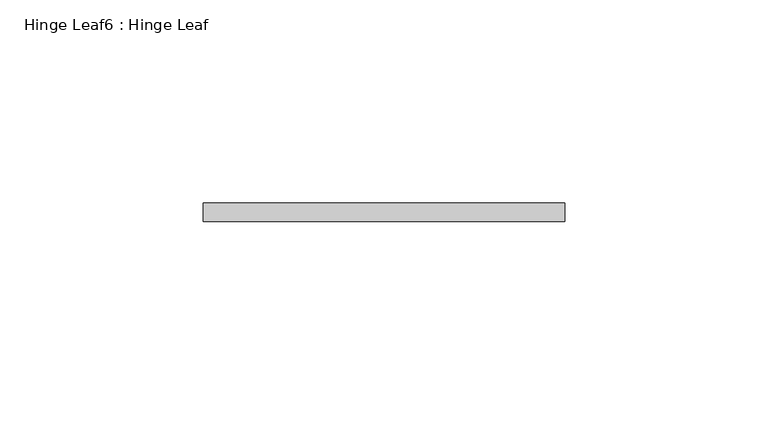
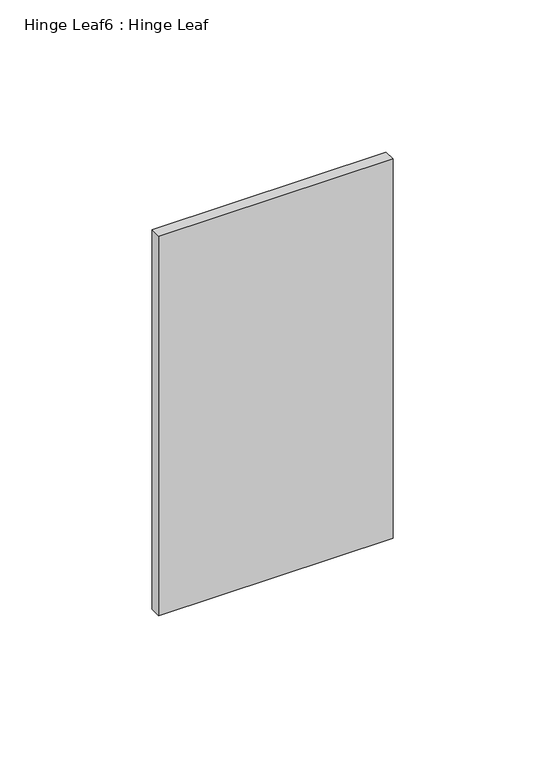
"""IFC4 building model written with IfcOpenShell, lengths in millimetres: proxy geometry, Hinge Leaf6 : Hinge Leaf."""

from ifc_helpers import new_model, si_unit, frame, origin, place, context, project, spatial, polyline, outline, extrude, source, transform, mapped, element, save


def hinge_leaf6_hinge_leaf_bcfbb292(model_context):
    return source(origin(), model_context, "Body", "SweptSolid", [
        extrude(outline(polyline([(587327.7934739, -533980.5883841), (587327.7934739, -533976.0163841), (587416.6934739, -533976.0163841), (587416.6934739, -533980.5883841), (587327.7934739, -533980.5883841)])), frame((0.0, 0.0, 311.15), z_axis=(0.0, 0.0, 1.0), x_axis=(1.0, 0.0, 0.0)), (0.0, 0.0, 1.0), 152.4),
    ])


if __name__ == "__main__":
    model = new_model("IFC4")
    model_context = context("Model", 3, world=origin())
    ifc_project = project(units=[si_unit("LENGTHUNIT", "METRE", prefix="MILLI")], contexts=[model_context])
    site = spatial("IfcSite", under=ifc_project)
    building = spatial("IfcBuilding", under=site)
    placement = place(None, origin())
    hinge_leaf6_hinge_leaf_shape = hinge_leaf6_hinge_leaf_bcfbb292(model_context)
    element("IfcBuildingElementProxy", 1, Name="Hinge Leaf6 : Hinge Leaf", ObjectType="Hinge Leaf6 : Hinge Leaf", at=placement, inside=building, context=model_context, shape_type="MappedRepresentation", body=[
        mapped(hinge_leaf6_hinge_leaf_shape, transform((0.0, 0.0, 0.0), x_axis=(1.0, 0.0, 0.0), y_axis=(0.0, 1.0, 0.0), z_axis=(0.0, 0.0, 1.0))),
    ])
    save(model, "model.ifc")

# Revit data of these elements
# Element 1 (IfcBuildingElementProxy, "Hinge Leaf6 : Hinge Leaf")
#   Materials on its faces: "6\"X6\" WELD-ON STL BUTT HINGE"
# Materials
#   "6\"X6\" WELD-ON STL BUTT HINGE": class "Metal", colour RGB 189 187 185, transparency 0, Description = "Carbon steel", Cost = 0
